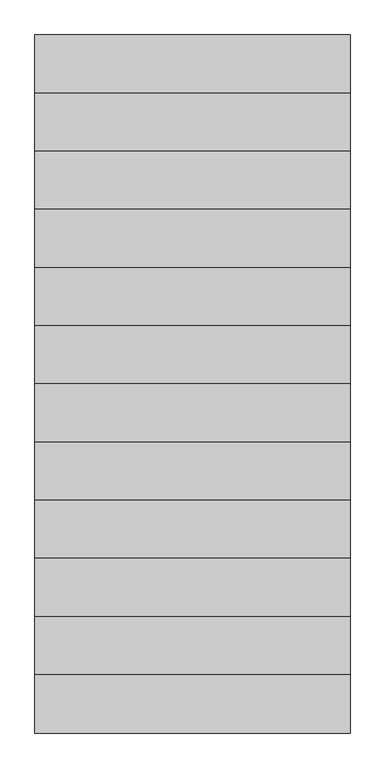
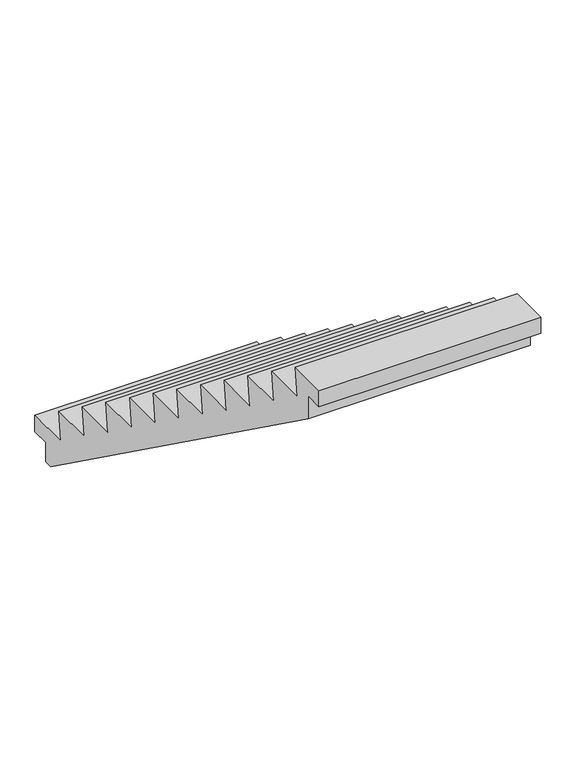
"""IFC4 building model written with IfcOpenShell, lengths in millimetres: stair geometry, NLRS_24_GM_LB_rechte steektrap prefab-AV_gen_rsf : prefab trap_gen__aant=11 b=1200 a=220 o=172.7 zonder bomen."""

from ifc_helpers import new_model, si_unit, frame, origin, place, context, project, spatial, polyline, outline, extrude, source, transform, mapped, element, save


def stair_c6ebb296(model_context):
    return source(origin(), model_context, "Body", "SweptSolid", [
        extrude(outline(polyline([(-2400.0, 1900.0), (-2420.0, 1727.2727273), (-2160.0, 1727.2727273), (-2180.0, 1554.5454545), (-1920.0, 1554.5454545), (-1940.0, 1381.8181818), (-1680.0, 1381.8181818), (-1700.0, 1209.0909091), (-1440.0, 1209.0909091), (-1460.0, 1036.3636364), (-1200.0, 1036.3636364), (-1220.0, 863.6363636), (-960.0, 863.6363636), (-980.0, 690.9090909), (-720.0, 690.9090909), (-740.0, 518.1818182), (-480.0, 518.1818182), (-500.0, 345.4545455), (-240.0, 345.4545455), (-260.0, 172.7272727), (0.0, 172.7272727), (-20.0, 0.0), (240.0, 0.0), (240.0, -100.0), (130.0, -100.0), (130.0, -220.0), (80.254966, -220.0), (-2530.0, 1658.5925892), (-2530.0, 1800.0), (-2640.0, 1800.0), (-2640.0, 1900.0), (-2400.0, 1900.0)])), frame((-650.0, 0.0, 0.0), z_axis=(1.0, 0.0, 0.0), x_axis=(0.0, 1.0, 0.0)), (0.0, 0.0, 1.0), 1300.0),
    ])


if __name__ == "__main__":
    model = new_model("IFC4")
    model_context = context("Model", 3, world=origin())
    ifc_project = project(units=[si_unit("LENGTHUNIT", "METRE", prefix="MILLI")], contexts=[model_context])
    site = spatial("IfcSite", under=ifc_project)
    building = spatial("IfcBuilding", under=site)
    placement = place(None, origin())
    stair_shape = stair_c6ebb296(model_context)
    element("IfcStair", 1, ObjectType="NLRS_24_GM_LB_rechte steektrap prefab-AV_gen_rsf : prefab trap_gen__aant=11 b=1200 a=220 o=172.7 zonder bomen", at=placement, inside=building, context=model_context, shape_type="MappedRepresentation", body=[
        mapped(stair_shape, transform((0.0, 0.0, 0.0), x_axis=(1.0, 0.0, 0.0), y_axis=(0.0, 1.0, 0.0), z_axis=(0.0, 0.0, 1.0))),
    ])
    save(model, "model.ifc")

# Revit data of these elements
# Type "NLRS_24_GM_LB_rechte steektrap prefab-AV_gen_rsf : prefab trap_gen__aant=11 b=1200 a=220 o=172.7 zonder bomen"
#   IfcExportAs = "IfcStair"
#   Type Comments = " "
#   Model = " "
#   Manufacturer = " "
#   Keynote = " "
#   Description = "rechte steektrap prefab\r\naant=11 b=1200 a=220 o=181,8\r\nzonder bomen"
#   Assembly Code = "24.11"
#   Aantrede onder = 240 mm
#   Width = 1300 mm
#   Wel diepte = 20 mm
#   Trapboom breedte = 0 mm
#   Thickness = 120 mm
#   Optrede onderste trede = 220 mm
#   NLRS_C_lengte = 2400 mm
#   Length = 2880 mm
#   Hoogte oplegnok onder = 100 mm
#   Hoogte oplegnok boven = 100 mm
#   Height = 1900 mm
#   Breedte oplegnok boven = 110 mm
#   BottomCalc = 0 mm
#   Actual Tread Depth = 240 mm
#   Actual Riser Height = 172.727 mm
#   Actual Number of Tread = 10
#   Actual Number of Risers = 11
#   Aantrede boven = 240 mm
#   Aantal treden max dertig = 11
#   Trapboom = no
#   Oplegnok onder = yes
#   NLRS_C_materiaal = NLRS_f2_beton prefab_gen_rsf
#   Default Elevation = 0
# Element 1 (IfcStair, "NLRS_24_GM_LB_rechte steektrap prefab-AV_gen_rsf : prefab trap_gen__aant=11 b=1200 a=220 o=172.7 zonder bomen")
#   Materials on its faces: "NLRS_f2_beton prefab_gen_rsf"
# Materials
#   "NLRS_f2_beton prefab_gen_rsf": class "F - Niet gebakken kunststeen", colour RGB 129 133 118, transparency 0, Keynote = "f2", Manufacturer = "Revit Standards Foundation", URL = "www.revitstandards.org", Description = "beton prefab", Cost = 0
